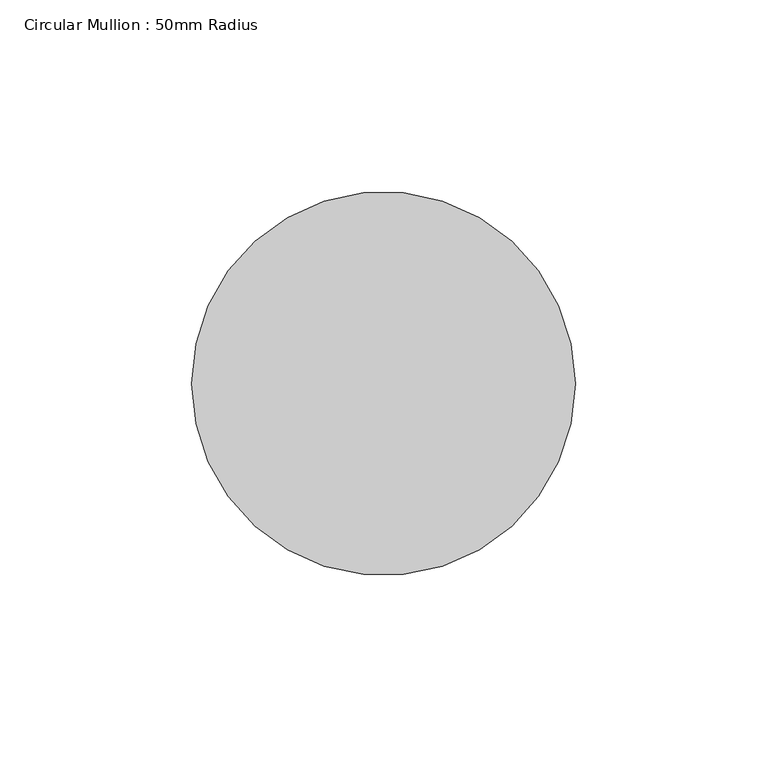
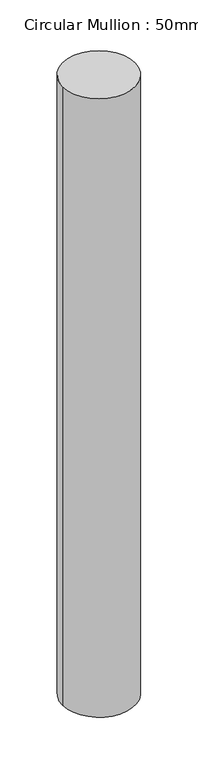
"""IFC4 building model written with IfcOpenShell, lengths in millimetres: member geometry, Circular Mullion : 50mm Radius."""

from ifc_helpers import new_model, si_unit, point, frame, origin, origin_2d, place, context, project, spatial, circle_curve, trimmed, segment, composite_curve, outline, extrude, source, transform, mapped, element, save


def circular_mullion_50mm_radius_96566982(model_context):
    return source(origin(), model_context, "Body", "SweptSolid", [
        extrude(outline(composite_curve([segment(trimmed(circle_curve(origin_2d(), 50.0), [point((50.0, 0.0))], [point((-50.0, 0.0))], False, "CARTESIAN"), True, "CONTINUOUS"), segment(trimmed(circle_curve(origin_2d(), 50.0), [point((-50.0, 0.0))], [point((50.0, 0.0))], False, "CARTESIAN"), True, "CONTINUOUS")], self_intersect=False)), frame((0.0, 0.0, -901.2453799), z_axis=(0.0, 0.0, 1.0), x_axis=(1.0, 0.0, 0.0)), (0.0, 0.0, 1.0), 901.2453799),
    ])


if __name__ == "__main__":
    model = new_model("IFC4")
    model_context = context("Model", 3, world=origin())
    ifc_project = project(units=[si_unit("LENGTHUNIT", "METRE", prefix="MILLI")], contexts=[model_context])
    site = spatial("IfcSite", under=ifc_project)
    building = spatial("IfcBuilding", under=site)
    placement = place(None, origin())
    circular_mullion_50mm_radius_shape = circular_mullion_50mm_radius_96566982(model_context)
    element("IfcMember", 1, ObjectType="Circular Mullion : 50mm Radius", at=placement, inside=building, context=model_context, shape_type="MappedRepresentation", body=[
        mapped(circular_mullion_50mm_radius_shape, transform((0.0, 0.0, 0.0), x_axis=(1.0, 0.0, 0.0), y_axis=(0.0, 1.0, 0.0), z_axis=(0.0, 0.0, 1.0))),
    ])
    save(model, "model.ifc")

# Revit data of these elements
# Type "Circular Mullion : 50mm Radius"
#   built-in parameter 1007350 = 0.164042 (stored number, unit not read)
# Element 1 (IfcMember, "Circular Mullion : 50mm Radius")
#   Materials on its faces: "Aluminium"
# Materials
#   "Aluminium": class "Metal", colour RGB 247 247 247, transparency 0, Description = "Aluminium 6061", Cost = 0
